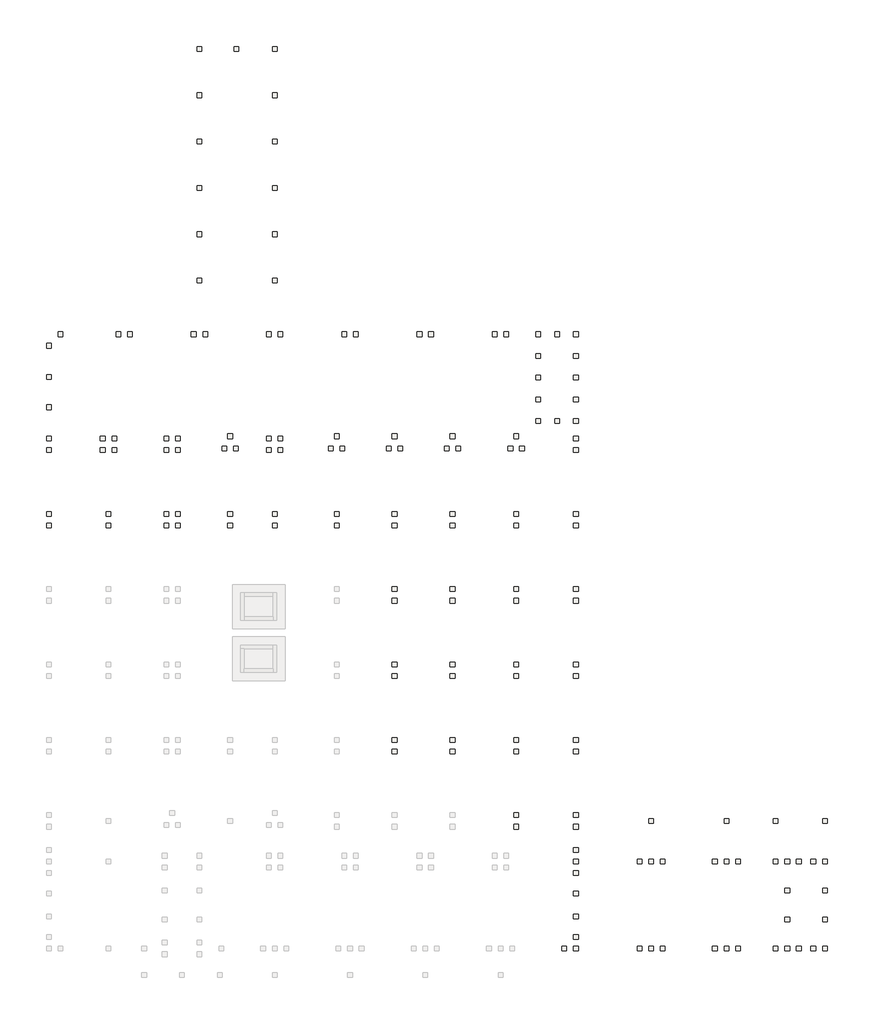
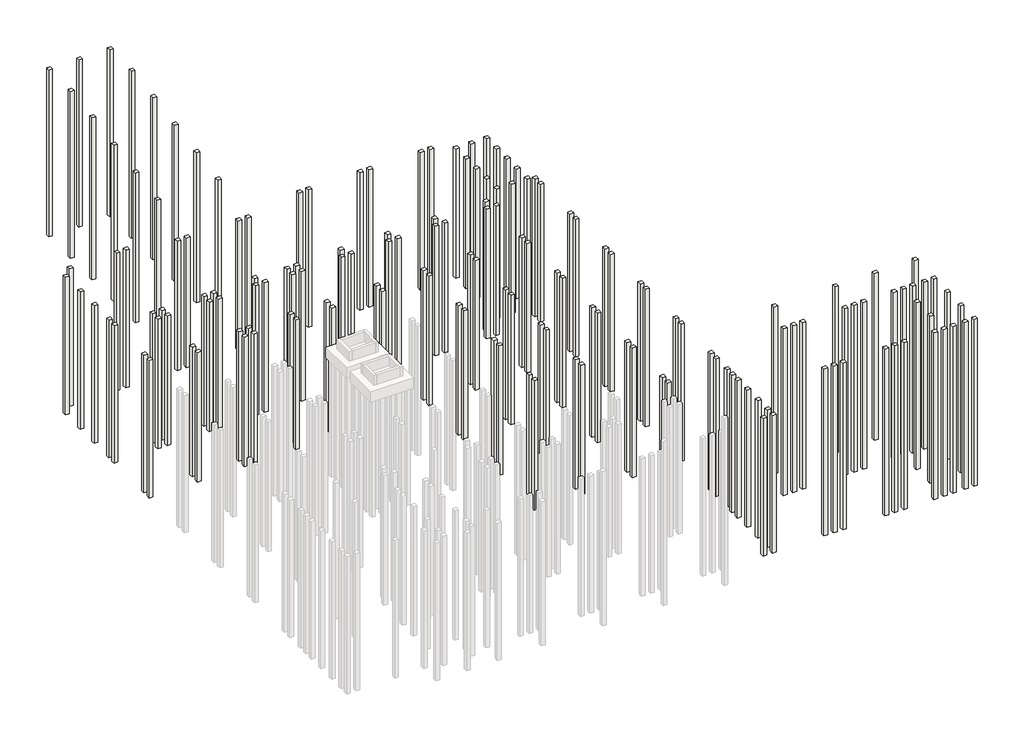
# Not in any storey, part 2 of 2: 160 slabs.
# Revit data of these elements (continued)
# Element 3 (IfcSlab, "NLRS_17_SFO_TLB_funderingspaal geheid beton prefab-AV-MMBPC_gen_rsf : heipaal beton prefab_gen__bxh 400x400") (continued)
#   Materials on its faces: "NLRS_f2_beton prefab_gen_rsf"
# Element 4 (IfcSlab, "NLRS_17_SFO_TLB_funderingspaal geheid beton prefab-AV-MMBPC_gen_rsf : heipaal beton prefab_gen__bxh 400x400")
#   IfcGUID = "10$Kfo5uPCAOPJEOo5LEs3"
#   Slanted Angle = 0.00°
#   NLRS_S_draagvermogen_trek = 0.00 kN
#   NLRS_S_draagvermogen_druk = 0.00 kN
#   Angle = 0.00°
#   IsExternal = yes
#   LoadBearing = yes
#   Slanted = 0
#   Phase Created = NLRS_nieuw
#   Materials on its faces: "NLRS_f2_beton prefab_gen_rsf"
# Element 5 (IfcSlab, "NLRS_17_SFO_TLB_funderingspaal geheid beton prefab-AV-MMBPC_gen_rsf : heipaal beton prefab_gen__bxh 400x400")
#   IfcGUID = "10$Kfo5uPCAOPJEOo5LEsU"
#   Slanted Angle = 0.00°
#   NLRS_S_draagvermogen_trek = 0.00 kN
#   NLRS_S_draagvermogen_druk = 0.00 kN
#   Angle = 0.00°
#   IsExternal = yes
#   LoadBearing = yes
#   Slanted = 0
#   Phase Created = NLRS_nieuw
#   Materials on its faces: "NLRS_f2_beton prefab_gen_rsf"
# Element 6 (IfcSlab, "NLRS_17_SFO_TLB_funderingspaal geheid beton prefab-AV-MMBPC_gen_rsf : heipaal beton prefab_gen__bxh 400x400")
#   IfcGUID = "10$Kfo5uPCAOPJEOo5LEsG"
#   Slanted Angle = 0.00°
#   NLRS_S_draagvermogen_trek = 0.00 kN
#   NLRS_S_draagvermogen_druk = 0.00 kN
#   Angle = 0.00°
#   IsExternal = yes
#   LoadBearing = yes
#   Slanted = 0
#   Phase Created = NLRS_nieuw
#   Materials on its faces: "NLRS_f2_beton prefab_gen_rsf"
# Element 7 (IfcSlab, "NLRS_17_SFO_TLB_funderingspaal geheid beton prefab-AV-MMBPC_gen_rsf : heipaal beton prefab_gen__bxh 400x400")
#   IfcGUID = "10$Kfo5uPCAOPJEOo5LEre"
#   Slanted Angle = 0.00°
#   NLRS_S_draagvermogen_trek = 0.00 kN
#   NLRS_S_draagvermogen_druk = 0.00 kN
#   Angle = 0.00°
#   IsExternal = yes
#   LoadBearing = yes
#   Slanted = 0
#   Phase Created = NLRS_nieuw
#   Materials on its faces: "NLRS_f2_beton prefab_gen_rsf"
# Element 8 (IfcSlab, "NLRS_17_SFO_TLB_funderingspaal geheid beton prefab-AV-MMBPC_gen_rsf : heipaal beton prefab_gen__bxh 400x400")
#   IfcGUID = "10$Kfo5uPCAOPJEOo5LErg"
#   Slanted Angle = 0.00°
#   NLRS_S_draagvermogen_trek = 0.00 kN
#   NLRS_S_draagvermogen_druk = 0.00 kN
#   Angle = 0.00°
#   IsExternal = yes
#   LoadBearing = yes
#   Slanted = 0
#   Phase Created = NLRS_nieuw
#   Materials on its faces: "NLRS_f2_beton prefab_gen_rsf"
# Element 9 (IfcSlab, "NLRS_17_SFO_TLB_funderingspaal geheid beton prefab-AV-MMBPC_gen_rsf : heipaal beton prefab_gen__bxh 400x400")
#   IfcGUID = "10$Kfo5uPCAOPJEOo5LEpb"
#   Slanted Angle = 0.00°
#   NLRS_S_draagvermogen_trek = 0.00 kN
#   NLRS_S_draagvermogen_druk = 0.00 kN
#   Angle = 0.00°
#   IsExternal = yes
#   LoadBearing = yes
#   Slanted = 0
#   Phase Created = NLRS_nieuw
#   Materials on its faces: "NLRS_f2_beton prefab_gen_rsf"
# Element 10 (IfcSlab, "NLRS_17_SFO_TLB_funderingspaal geheid beton prefab-AV-MMBPC_gen_rsf : heipaal beton prefab_gen__bxh 400x400")
#   IfcGUID = "10$Kfo5uPCAOPJEOo5LEpd"
#   Slanted Angle = 0.00°
#   NLRS_S_draagvermogen_trek = 0.00 kN
#   NLRS_S_draagvermogen_druk = 0.00 kN
#   Angle = 0.00°
#   IsExternal = yes
#   LoadBearing = yes
#   Slanted = 0
#   Phase Created = NLRS_nieuw
#   Materials on its faces: "NLRS_f2_beton prefab_gen_rsf"
# Element 11 (IfcSlab, "NLRS_17_SFO_TLB_funderingspaal geheid beton prefab-AV-MMBPC_gen_rsf : heipaal beton prefab_gen__bxh 400x400")
#   IfcGUID = "10$Kfo5uPCAOPJEOo5LEpz"
#   Slanted Angle = 0.00°
#   NLRS_S_draagvermogen_trek = 0.00 kN
#   NLRS_S_draagvermogen_druk = 0.00 kN
#   Angle = 0.00°
#   IsExternal = yes
#   LoadBearing = yes
#   Slanted = 0
#   Phase Created = NLRS_nieuw
#   Materials on its faces: "NLRS_f2_beton prefab_gen_rsf"
# Element 12 (IfcSlab, "NLRS_17_SFO_TLB_funderingspaal geheid beton prefab-AV-MMBPC_gen_rsf : heipaal beton prefab_gen__bxh 400x400")
#   IfcGUID = "10$Kfo5uPCAOPJEOo5LEp$"
#   Slanted Angle = 0.00°
#   NLRS_S_draagvermogen_trek = 0.00 kN
#   NLRS_S_draagvermogen_druk = 0.00 kN
#   Angle = 0.00°
#   IsExternal = yes
#   LoadBearing = yes
#   Slanted = 0
#   Phase Created = NLRS_nieuw
#   Materials on its faces: "NLRS_f2_beton prefab_gen_rsf"
# Element 13 (IfcSlab, "NLRS_17_SFO_TLB_funderingspaal geheid beton prefab-AV-MMBPC_gen_rsf : heipaal beton prefab_gen__bxh 400x400")
#   IfcGUID = "10$Kfo5uPCAOPJEOo5LFTh"
#   Slanted Angle = 0.00°
#   NLRS_S_draagvermogen_trek = 0.00 kN
#   NLRS_S_draagvermogen_druk = 0.00 kN
#   Angle = 0.00°
#   IsExternal = yes
#   LoadBearing = yes
#   Slanted = 0
#   Phase Created = NLRS_nieuw
#   Materials on its faces: "NLRS_f2_beton prefab_gen_rsf"
# Element 14 (IfcSlab, "NLRS_17_SFO_TLB_funderingspaal geheid beton prefab-AV-MMBPC_gen_rsf : heipaal beton prefab_gen__bxh 400x400")
#   IfcGUID = "10$Kfo5uPCAOPJEOo5LFSD"
#   Slanted Angle = 0.00°
#   NLRS_S_draagvermogen_trek = 0.00 kN
#   NLRS_S_draagvermogen_druk = 0.00 kN
#   Angle = 0.00°
#   IsExternal = yes
#   LoadBearing = yes
#   Slanted = 0
#   Phase Created = NLRS_nieuw
#   Materials on its faces: "NLRS_f2_beton prefab_gen_rsf"
# Element 15 (IfcSlab, "NLRS_17_SFO_TLB_funderingspaal geheid beton prefab-AV-MMBPC_gen_rsf : heipaal beton prefab_gen__bxh 400x400")
#   IfcGUID = "10$Kfo5uPCAOPJEOo5LFSk"
#   Slanted Angle = 0.00°
#   NLRS_S_draagvermogen_trek = 0.00 kN
#   NLRS_S_draagvermogen_druk = 0.00 kN
#   Angle = 0.00°
#   IsExternal = yes
#   LoadBearing = yes
#   Slanted = 0
#   Phase Created = NLRS_nieuw
#   Materials on its faces: "NLRS_f2_beton prefab_gen_rsf"
# Element 16 (IfcSlab, "NLRS_17_SFO_TLB_funderingspaal geheid beton prefab-AV-MMBPC_gen_rsf : heipaal beton prefab_gen__bxh 400x400")
#   IfcGUID = "10$Kfo5uPCAOPJEOo5LFSv"
#   Slanted Angle = 0.00°
#   NLRS_S_draagvermogen_trek = 0.00 kN
#   NLRS_S_draagvermogen_druk = 0.00 kN
#   Angle = 0.00°
#   IsExternal = yes
#   LoadBearing = yes
#   Slanted = 0
#   Phase Created = NLRS_nieuw
#   Materials on its faces: "NLRS_f2_beton prefab_gen_rsf"
# Element 17 (IfcSlab, "NLRS_17_SFO_TLB_funderingspaal geheid beton prefab-AV-MMBPC_gen_rsf : heipaal beton prefab_gen__bxh 400x400")
#   IfcGUID = "10$Kfo5uPCAOPJEOo5LFSs"
#   Slanted Angle = 0.00°
#   NLRS_S_draagvermogen_trek = 0.00 kN
#   NLRS_S_draagvermogen_druk = 0.00 kN
#   Angle = 0.00°
#   IsExternal = yes
#   LoadBearing = yes
#   Slanted = 0
#   Phase Created = NLRS_nieuw
#   Materials on its faces: "NLRS_f2_beton prefab_gen_rsf"
# Element 18 (IfcSlab, "NLRS_17_SFO_TLB_funderingspaal geheid beton prefab-AV-MMBPC_gen_rsf : heipaal beton prefab_gen__bxh 400x400")
#   IfcGUID = "10$Kfo5uPCAOPJEOo5LFR1"
#   Slanted Angle = 0.00°
#   NLRS_S_draagvermogen_trek = 0.00 kN
#   NLRS_S_draagvermogen_druk = 0.00 kN
#   Angle = 0.00°
#   IsExternal = yes
#   LoadBearing = yes
#   Slanted = 0
#   Phase Created = NLRS_nieuw
#   Materials on its faces: "NLRS_f2_beton prefab_gen_rsf"
# Element 19 (IfcSlab, "NLRS_17_SFO_TLB_funderingspaal geheid beton prefab-AV-MMBPC_gen_rsf : heipaal beton prefab_gen__bxh 400x400")
#   IfcGUID = "10$Kfo5uPCAOPJEOo5LFQO"
#   Slanted Angle = 0.00°
#   NLRS_S_draagvermogen_trek = 0.00 kN
#   NLRS_S_draagvermogen_druk = 0.00 kN
#   Angle = 0.00°
#   IsExternal = yes
#   LoadBearing = yes
#   Slanted = 0
#   Phase Created = NLRS_nieuw
#   Materials on its faces: "NLRS_f2_beton prefab_gen_rsf"
# Element 20 (IfcSlab, "NLRS_17_SFO_TLB_funderingspaal geheid beton prefab-AV-MMBPC_gen_rsf : heipaal beton prefab_gen__bxh 400x400")
#   IfcGUID = "10$Kfo5uPCAOPJEOo5LFQJ"
#   Slanted Angle = 0.00°
#   NLRS_S_draagvermogen_trek = 0.00 kN
#   NLRS_S_draagvermogen_druk = 0.00 kN
#   Angle = 0.00°
#   IsExternal = yes
#   LoadBearing = yes
#   Slanted = 0
#   Phase Created = NLRS_nieuw
#   Materials on its faces: "NLRS_f2_beton prefab_gen_rsf"
# Element 21 (IfcSlab, "NLRS_17_SFO_TLB_funderingspaal geheid beton prefab-AV-MMBPC_gen_rsf : heipaal beton prefab_gen__bxh 400x400")
#   IfcGUID = "10$Kfo5uPCAOPJEOo5LFQk"
#   Slanted Angle = 0.00°
#   NLRS_S_draagvermogen_trek = 0.00 kN
#   NLRS_S_draagvermogen_druk = 0.00 kN
#   Angle = 0.00°
#   IsExternal = yes
#   LoadBearing = yes
#   Slanted = 0
#   Phase Created = NLRS_nieuw
#   Materials on its faces: "NLRS_f2_beton prefab_gen_rsf"
# Element 22 (IfcSlab, "NLRS_17_SFO_TLB_funderingspaal geheid beton prefab-AV-MMBPC_gen_rsf : heipaal beton prefab_gen__bxh 400x400")
#   IfcGUID = "10$Kfo5uPCAOPJEOo5LFPx"
#   Slanted Angle = 0.00°
#   NLRS_S_draagvermogen_trek = 0.00 kN
#   NLRS_S_draagvermogen_druk = 0.00 kN
#   Angle = 0.00°
#   IsExternal = yes
#   LoadBearing = yes
#   Slanted = 0
#   Phase Created = NLRS_nieuw
#   Materials on its faces: "NLRS_f2_beton prefab_gen_rsf"
# Element 23 (IfcSlab, "NLRS_17_SFO_TLB_funderingspaal geheid beton prefab-AV-MMBPC_gen_rsf : heipaal beton prefab_gen__bxh 400x400")
#   IfcGUID = "10$Kfo5uPCAOPJEOo5LFOK"
#   Slanted Angle = 0.00°
#   NLRS_S_draagvermogen_trek = 0.00 kN
#   NLRS_S_draagvermogen_druk = 0.00 kN
#   Angle = 0.00°
#   IsExternal = yes
#   LoadBearing = yes
#   Slanted = 0
#   Phase Created = NLRS_nieuw
#   Materials on its faces: "NLRS_f2_beton prefab_gen_rsf"
# Element 24 (IfcSlab, "NLRS_17_SFO_TLB_funderingspaal geheid beton prefab-AV-MMBPC_gen_rsf : heipaal beton prefab_gen__bxh 400x400")
#   IfcGUID = "10$Kfo5uPCAOPJEOo5LFOl"
#   Slanted Angle = 0.00°
#   NLRS_S_draagvermogen_trek = 0.00 kN
#   NLRS_S_draagvermogen_druk = 0.00 kN
#   Angle = 0.00°
#   IsExternal = yes
#   LoadBearing = yes
#   Slanted = 0
#   Phase Created = NLRS_nieuw
#   Materials on its faces: "NLRS_f2_beton prefab_gen_rsf"
# Element 25 (IfcSlab, "NLRS_17_SFO_TLB_funderingspaal geheid beton prefab-AV-MMBPC_gen_rsf : heipaal beton prefab_gen__bxh 400x400")
#   IfcGUID = "3loy75XKz2Rw4dS8JWiamE"
#   Slanted Angle = 0.00°
#   NLRS_S_draagvermogen_trek = 0.00 kN
#   NLRS_S_draagvermogen_druk = 0.00 kN
#   Angle = 0.00°
#   IsExternal = yes
#   LoadBearing = yes
#   Slanted = 0
#   Phase Created = NLRS_nieuw
#   Materials on its faces: "NLRS_f2_beton prefab_gen_rsf"
# Element 26 (IfcSlab, "NLRS_17_SFO_TLB_funderingspaal geheid beton prefab-AV-MMBPC_gen_rsf : heipaal beton prefab_gen__bxh 400x400")
#   IfcGUID = "3loy75XKz2Rw4dS8JWiamC"
#   Slanted Angle = 0.00°
#   NLRS_S_draagvermogen_trek = 0.00 kN
#   NLRS_S_draagvermogen_druk = 0.00 kN
#   Angle = 0.00°
#   IsExternal = yes
#   LoadBearing = yes
#   Slanted = 0
#   Phase Created = NLRS_nieuw
#   Materials on its faces: "NLRS_f2_beton prefab_gen_rsf"
# Element 27 (IfcSlab, "NLRS_17_SFO_TLB_funderingspaal geheid beton prefab-AV-MMBPC_gen_rsf : heipaal beton prefab_gen__bxh 400x400")
#   IfcGUID = "3loy75XKz2Rw4dS8JWiamv"
#   Slanted Angle = 0.00°
#   NLRS_S_draagvermogen_trek = 0.00 kN
#   NLRS_S_draagvermogen_druk = 0.00 kN
#   Angle = 0.00°
#   IsExternal = yes
#   LoadBearing = yes
#   Slanted = 0
#   Phase Created = NLRS_nieuw
#   Materials on its faces: "NLRS_f2_beton prefab_gen_rsf"
# Element 28 (IfcSlab, "NLRS_17_SFO_TLB_funderingspaal geheid beton prefab-AV-MMBPC_gen_rsf : heipaal beton prefab_gen__bxh 400x400")
#   IfcGUID = "3loy75XKz2Rw4dS8JWiam$"
#   Slanted Angle = 0.00°
#   NLRS_S_draagvermogen_trek = 0.00 kN
#   NLRS_S_draagvermogen_druk = 0.00 kN
#   Angle = 0.00°
#   IsExternal = yes
#   LoadBearing = yes
#   Slanted = 0
#   Phase Created = NLRS_nieuw
#   Materials on its faces: "NLRS_f2_beton prefab_gen_rsf"
# Element 29 (IfcSlab, "NLRS_17_SFO_TLB_funderingspaal geheid beton prefab-AV-MMBPC_gen_rsf : heipaal beton prefab_gen__bxh 400x400")
#   IfcGUID = "3loy75XKz2Rw4dS8JWiama"
#   Slanted Angle = 0.00°
#   NLRS_S_draagvermogen_trek = 0.00 kN
#   NLRS_S_draagvermogen_druk = 0.00 kN
#   Angle = 0.00°
#   IsExternal = yes
#   LoadBearing = yes
#   Slanted = 0
#   Phase Created = NLRS_nieuw
#   Materials on its faces: "NLRS_f2_beton prefab_gen_rsf"
# Element 30 (IfcSlab, "NLRS_17_SFO_TLB_funderingspaal geheid beton prefab-AV-MMBPC_gen_rsf : heipaal beton prefab_gen__bxh 400x400")
#   IfcGUID = "3loy75XKz2Rw4dS8JWiamg"
#   Slanted Angle = 0.00°
#   NLRS_S_draagvermogen_trek = 0.00 kN
#   NLRS_S_draagvermogen_druk = 0.00 kN
#   Angle = 0.00°
#   IsExternal = yes
#   LoadBearing = yes
#   Slanted = 0
#   Phase Created = NLRS_nieuw
#   Materials on its faces: "NLRS_f2_beton prefab_gen_rsf"
# Element 31 (IfcSlab, "NLRS_17_SFO_TLB_funderingspaal geheid beton prefab-AV-MMBPC_gen_rsf : heipaal beton prefab_gen__bxh 400x400")
#   IfcGUID = "3loy75XKz2Rw4dS8JWiapN"
#   Slanted Angle = 0.00°
#   NLRS_S_draagvermogen_trek = 0.00 kN
#   NLRS_S_draagvermogen_druk = 0.00 kN
#   Angle = 0.00°
#   IsExternal = yes
#   LoadBearing = yes
#   Slanted = 0
#   Phase Created = NLRS_nieuw
#   Materials on its faces: "NLRS_f2_beton prefab_gen_rsf"
# Element 32 (IfcSlab, "NLRS_17_SFO_TLB_funderingspaal geheid beton prefab-AV-MMBPC_gen_rsf : heipaal beton prefab_gen__bxh 400x400")
#   IfcGUID = "3loy75XKz2Rw4dS8JWiapL"
#   Slanted Angle = 0.00°
#   NLRS_S_draagvermogen_trek = 0.00 kN
#   NLRS_S_draagvermogen_druk = 0.00 kN
#   Angle = 0.00°
#   IsExternal = yes
#   LoadBearing = yes
#   Slanted = 0
#   Phase Created = NLRS_nieuw
#   Materials on its faces: "NLRS_f2_beton prefab_gen_rsf"
# Element 33 (IfcSlab, "NLRS_17_SFO_TLB_funderingspaal geheid beton prefab-AV-MMBPC_gen_rsf : heipaal beton prefab_gen__bxh 400x400")
#   IfcGUID = "3loy75XKz2Rw4dS8JWiap2"
#   Slanted Angle = 0.00°
#   NLRS_S_draagvermogen_trek = 0.00 kN
#   NLRS_S_draagvermogen_druk = 0.00 kN
#   Angle = 0.00°
#   IsExternal = yes
#   LoadBearing = yes
#   Slanted = 0
#   Phase Created = NLRS_nieuw
#   Materials on its faces: "NLRS_f2_beton prefab_gen_rsf"
# Element 34 (IfcSlab, "NLRS_17_SFO_TLB_funderingspaal geheid beton prefab-AV-MMBPC_gen_rsf : heipaal beton prefab_gen__bxh 400x400")
#   IfcGUID = "3loy75XKz2Rw4dS8JWiap0"
#   Slanted Angle = 0.00°
#   NLRS_S_draagvermogen_trek = 0.00 kN
#   NLRS_S_draagvermogen_druk = 0.00 kN
#   Angle = 0.00°
#   IsExternal = yes
#   LoadBearing = yes
#   Slanted = 0
#   Phase Created = NLRS_nieuw
#   Materials on its faces: "NLRS_f2_beton prefab_gen_rsf"
# Element 35 (IfcSlab, "NLRS_17_SFO_TLB_funderingspaal geheid beton prefab-AV-MMBPC_gen_rsf : heipaal beton prefab_gen__bxh 400x400")
#   IfcGUID = "3loy75XKz2Rw4dS8JWiapD"
#   Slanted Angle = 0.00°
#   NLRS_S_draagvermogen_trek = 0.00 kN
#   NLRS_S_draagvermogen_druk = 0.00 kN
#   Angle = 0.00°
#   IsExternal = yes
#   LoadBearing = yes
#   Slanted = 0
#   Phase Created = NLRS_nieuw
#   Materials on its faces: "NLRS_f2_beton prefab_gen_rsf"
# Element 36 (IfcSlab, "NLRS_17_SFO_TLB_funderingspaal geheid beton prefab-AV-MMBPC_gen_rsf : heipaal beton prefab_gen__bxh 400x400")
#   IfcGUID = "3loy75XKz2Rw4dS8JWiapp"
#   Slanted Angle = 0.00°
#   NLRS_S_draagvermogen_trek = 0.00 kN
#   NLRS_S_draagvermogen_druk = 0.00 kN
#   Angle = 0.00°
#   IsExternal = yes
#   LoadBearing = yes
#   Slanted = 0
#   Phase Created = NLRS_nieuw
#   Materials on its faces: "NLRS_f2_beton prefab_gen_rsf"
# Element 37 (IfcSlab, "NLRS_17_SFO_TLB_funderingspaal geheid beton prefab-AV-MMBPC_gen_rsf : heipaal beton prefab_gen__bxh 400x400")
#   IfcGUID = "3loy75XKz2Rw4dS8JWiao6"
#   Slanted Angle = 0.00°
#   NLRS_S_draagvermogen_trek = 0.00 kN
#   NLRS_S_draagvermogen_druk = 0.00 kN
#   Angle = 0.00°
#   IsExternal = yes
#   LoadBearing = yes
#   Slanted = 0
#   Phase Created = NLRS_nieuw
#   Materials on its faces: "NLRS_f2_beton prefab_gen_rsf"
# Element 38 (IfcSlab, "NLRS_17_SFO_TLB_funderingspaal geheid beton prefab-AV-MMBPC_gen_rsf : heipaal beton prefab_gen__bxh 400x400")
#   IfcGUID = "3loy75XKz2Rw4dS8JWiao4"
#   Slanted Angle = 0.00°
#   NLRS_S_draagvermogen_trek = 0.00 kN
#   NLRS_S_draagvermogen_druk = 0.00 kN
#   Angle = 0.00°
#   IsExternal = yes
#   LoadBearing = yes
#   Slanted = 0
#   Phase Created = NLRS_nieuw
#   Materials on its faces: "NLRS_f2_beton prefab_gen_rsf"
# Element 39 (IfcSlab, "NLRS_17_SFO_TLB_funderingspaal geheid beton prefab-AV-MMBPC_gen_rsf : heipaal beton prefab_gen__bxh 400x400")
#   IfcGUID = "3loy75XKz2Rw4dS8JWiaon"
#   Slanted Angle = 0.00°
#   NLRS_S_draagvermogen_trek = 0.00 kN
#   NLRS_S_draagvermogen_druk = 0.00 kN
#   Angle = 0.00°
#   IsExternal = yes
#   LoadBearing = yes
#   Slanted = 0
#   Phase Created = NLRS_nieuw
#   Materials on its faces: "NLRS_f2_beton prefab_gen_rsf"
# Element 40 (IfcSlab, "NLRS_17_SFO_TLB_funderingspaal geheid beton prefab-AV-MMBPC_gen_rsf : heipaal beton prefab_gen__bxh 400x400")
#   IfcGUID = "3loy75XKz2Rw4dS8JWiaot"
#   Slanted Angle = 0.00°
#   NLRS_S_draagvermogen_trek = 0.00 kN
#   NLRS_S_draagvermogen_druk = 0.00 kN
#   Angle = 0.00°
#   IsExternal = yes
#   LoadBearing = yes
#   Slanted = 0
#   Phase Created = NLRS_nieuw
#   Materials on its faces: "NLRS_f2_beton prefab_gen_rsf"
# Element 41 (IfcSlab, "NLRS_17_SFO_TLB_funderingspaal geheid beton prefab-AV-MMBPC_gen_rsf : heipaal beton prefab_gen__bxh 400x400")
#   IfcGUID = "3loy75XKz2Rw4dS8JWiaoy"
#   Slanted Angle = 0.00°
#   NLRS_S_draagvermogen_trek = 0.00 kN
#   NLRS_S_draagvermogen_druk = 0.00 kN
#   Angle = 0.00°
#   IsExternal = yes
#   LoadBearing = yes
#   Slanted = 0
#   Phase Created = NLRS_nieuw
#   Materials on its faces: "NLRS_f2_beton prefab_gen_rsf"
# Element 42 (IfcSlab, "NLRS_17_SFO_TLB_funderingspaal geheid beton prefab-AV-MMBPC_gen_rsf : heipaal beton prefab_gen__bxh 400x400")
#   IfcGUID = "3loy75XKz2Rw4dS8JWiaoY"
#   Slanted Angle = 0.00°
#   NLRS_S_draagvermogen_trek = 0.00 kN
#   NLRS_S_draagvermogen_druk = 0.00 kN
#   Angle = 0.00°
#   IsExternal = yes
#   LoadBearing = yes
#   Slanted = 0
#   Phase Created = NLRS_nieuw
#   Materials on its faces: "NLRS_f2_beton prefab_gen_rsf"
# Element 43 (IfcSlab, "NLRS_17_SFO_TLB_funderingspaal geheid beton prefab-AV-MMBPC_gen_rsf : heipaal beton prefab_gen__bxh 400x400")
#   IfcGUID = "3loy75XKz2Rw4dS8JWiaol"
#   Slanted Angle = 0.00°
#   NLRS_S_draagvermogen_trek = 0.00 kN
#   NLRS_S_draagvermogen_druk = 0.00 kN
#   Angle = 0.00°
#   IsExternal = yes
#   LoadBearing = yes
#   Slanted = 0
#   Phase Created = NLRS_nieuw
#   Materials on its faces: "NLRS_f2_beton prefab_gen_rsf"
# Element 44 (IfcSlab, "NLRS_17_SFO_TLB_funderingspaal geheid beton prefab-AV-MMBPC_gen_rsf : heipaal beton prefab_gen__bxh 400x400")
#   IfcGUID = "3loy75XKz2Rw4dS8JWiaoj"
#   Slanted Angle = 0.00°
#   NLRS_S_draagvermogen_trek = 0.00 kN
#   NLRS_S_draagvermogen_druk = 0.00 kN
#   Angle = 0.00°
#   IsExternal = yes
#   LoadBearing = yes
#   Slanted = 0
#   Phase Created = NLRS_nieuw
#   Materials on its faces: "NLRS_f2_beton prefab_gen_rsf"
# Element 45 (IfcSlab, "NLRS_17_SFO_TLB_funderingspaal geheid beton prefab-AV-MMBPC_gen_rsf : heipaal beton prefab_gen__bxh 400x400")
#   IfcGUID = "3loy75XKz2Rw4dS8JWiarQ"
#   Slanted Angle = 0.00°
#   NLRS_S_draagvermogen_trek = 0.00 kN
#   NLRS_S_draagvermogen_druk = 0.00 kN
#   Angle = 0.00°
#   IsExternal = yes
#   LoadBearing = yes
#   Slanted = 0
#   Phase Created = NLRS_nieuw
#   Materials on its faces: "NLRS_f2_beton prefab_gen_rsf"
# Element 46 (IfcSlab, "NLRS_17_SFO_TLB_funderingspaal geheid beton prefab-AV-MMBPC_gen_rsf : heipaal beton prefab_gen__bxh 400x400")
#   IfcGUID = "3loy75XKz2Rw4dS8JWiarO"
#   Slanted Angle = 0.00°
#   NLRS_S_draagvermogen_trek = 0.00 kN
#   NLRS_S_draagvermogen_druk = 0.00 kN
#   Angle = 0.00°
#   IsExternal = yes
#   LoadBearing = yes
#   Slanted = 0
#   Phase Created = NLRS_nieuw
#   Materials on its faces: "NLRS_f2_beton prefab_gen_rsf"
# Element 47 (IfcSlab, "NLRS_17_SFO_TLB_funderingspaal geheid beton prefab-AV-MMBPC_gen_rsf : heipaal beton prefab_gen__bxh 400x400")
#   IfcGUID = "3loy75XKz2Rw4dS8JWiar5"
#   Slanted Angle = 0.00°
#   NLRS_S_draagvermogen_trek = 0.00 kN
#   NLRS_S_draagvermogen_druk = 0.00 kN
#   Angle = 0.00°
#   IsExternal = yes
#   LoadBearing = yes
#   Slanted = 0
#   Phase Created = NLRS_nieuw
#   Materials on its faces: "NLRS_f2_beton prefab_gen_rsf"
# Element 48 (IfcSlab, "NLRS_17_SFO_TLB_funderingspaal geheid beton prefab-AV-MMBPC_gen_rsf : heipaal beton prefab_gen__bxh 400x400")
#   IfcGUID = "3loy75XKz2Rw4dS8JWiarB"
#   Slanted Angle = 0.00°
#   NLRS_S_draagvermogen_trek = 0.00 kN
#   NLRS_S_draagvermogen_druk = 0.00 kN
#   Angle = 0.00°
#   IsExternal = yes
#   LoadBearing = yes
#   Slanted = 0
#   Phase Created = NLRS_nieuw
#   Materials on its faces: "NLRS_f2_beton prefab_gen_rsf"
# Element 49 (IfcSlab, "NLRS_17_SFO_TLB_funderingspaal geheid beton prefab-AV-MMBPC_gen_rsf : heipaal beton prefab_gen__bxh 400x400")
#   IfcGUID = "3loy75XKz2Rw4dS8JWiarm"
#   Slanted Angle = 0.00°
#   NLRS_S_draagvermogen_trek = 0.00 kN
#   NLRS_S_draagvermogen_druk = 0.00 kN
#   Angle = 0.00°
#   IsExternal = yes
#   LoadBearing = yes
#   Slanted = 0
#   Phase Created = NLRS_nieuw
#   Materials on its faces: "NLRS_f2_beton prefab_gen_rsf"
# Element 50 (IfcSlab, "NLRS_17_SFO_TLB_funderingspaal geheid beton prefab-AV-MMBPC_gen_rsf : heipaal beton prefab_gen__bxh 400x400")
#   IfcGUID = "3loy75XKz2Rw4dS8JWiars"
#   Slanted Angle = 0.00°
#   NLRS_S_draagvermogen_trek = 0.00 kN
#   NLRS_S_draagvermogen_druk = 0.00 kN
#   Angle = 0.00°
#   IsExternal = yes
#   LoadBearing = yes
#   Slanted = 0
#   Phase Created = NLRS_nieuw
#   Materials on its faces: "NLRS_f2_beton prefab_gen_rsf"
# Element 51 (IfcSlab, "NLRS_17_SFO_TLB_funderingspaal geheid beton prefab-AV-MMBPC_gen_rsf : heipaal beton prefab_gen__bxh 400x400")
#   IfcGUID = "3loy75XKz2Rw4dS8JWia96"
#   Slanted Angle = 0.00°
#   NLRS_S_draagvermogen_trek = 0.00 kN
#   NLRS_S_draagvermogen_druk = 0.00 kN
#   Angle = 0.00°
#   IsExternal = yes
#   LoadBearing = yes
#   Slanted = 0
#   Phase Created = NLRS_nieuw
#   Materials on its faces: "NLRS_f2_beton prefab_gen_rsf"
# Element 52 (IfcSlab, "NLRS_17_SFO_TLB_funderingspaal geheid beton prefab-AV-MMBPC_gen_rsf : heipaal beton prefab_gen__bxh 400x400")
#   IfcGUID = "3loy75XKz2Rw4dS8JWia94"
#   Slanted Angle = 0.00°
#   NLRS_S_draagvermogen_trek = 0.00 kN
#   NLRS_S_draagvermogen_druk = 0.00 kN
#   Angle = 0.00°
#   IsExternal = yes
#   LoadBearing = yes
#   Slanted = 0
#   Phase Created = NLRS_nieuw
#   Materials on its faces: "NLRS_f2_beton prefab_gen_rsf"
# Element 53 (IfcSlab, "NLRS_17_SFO_TLB_funderingspaal geheid beton prefab-AV-MMBPC_gen_rsf : heipaal beton prefab_gen__bxh 400x400")
#   IfcGUID = "3loy75XKz2Rw4dS8JWia9A"
#   Slanted Angle = 0.00°
#   NLRS_S_draagvermogen_trek = 0.00 kN
#   NLRS_S_draagvermogen_druk = 0.00 kN
#   Angle = 0.00°
#   IsExternal = yes
#   LoadBearing = yes
#   Slanted = 0
#   Phase Created = NLRS_nieuw
#   Materials on its faces: "NLRS_f2_beton prefab_gen_rsf"
# Element 54 (IfcSlab, "NLRS_17_SFO_TLB_funderingspaal geheid beton prefab-AV-MMBPC_gen_rsf : heipaal beton prefab_gen__bxh 400x400")
#   IfcGUID = "3loy75XKz2Rw4dS8JWia98"
#   Slanted Angle = 0.00°
#   NLRS_S_draagvermogen_trek = 0.00 kN
#   NLRS_S_draagvermogen_druk = 0.00 kN
#   Angle = 0.00°
#   IsExternal = yes
#   LoadBearing = yes
#   Slanted = 0
#   Phase Created = NLRS_nieuw
#   Materials on its faces: "NLRS_f2_beton prefab_gen_rsf"
# Element 55 (IfcSlab, "NLRS_17_SFO_TLB_funderingspaal geheid beton prefab-AV-MMBPC_gen_rsf : heipaal beton prefab_gen__bxh 400x400")
#   IfcGUID = "3loy75XKz2Rw4dS8JWia9l"
#   Slanted Angle = 0.00°
#   NLRS_S_draagvermogen_trek = 0.00 kN
#   NLRS_S_draagvermogen_druk = 0.00 kN
#   Angle = 0.00°
#   IsExternal = yes
#   LoadBearing = yes
#   Slanted = 0
#   Phase Created = NLRS_nieuw
#   Materials on its faces: "NLRS_f2_beton prefab_gen_rsf"
# Element 56 (IfcSlab, "NLRS_17_SFO_TLB_funderingspaal geheid beton prefab-AV-MMBPC_gen_rsf : heipaal beton prefab_gen__bxh 400x400")
#   IfcGUID = "3loy75XKz2Rw4dS8JWia9j"
#   Slanted Angle = 0.00°
#   NLRS_S_draagvermogen_trek = 0.00 kN
#   NLRS_S_draagvermogen_druk = 0.00 kN
#   Angle = 0.00°
#   IsExternal = yes
#   LoadBearing = yes
#   Slanted = 0
#   Phase Created = NLRS_nieuw
#   Materials on its faces: "NLRS_f2_beton prefab_gen_rsf"
# Element 57 (IfcSlab, "NLRS_17_SFO_TLB_funderingspaal geheid beton prefab-AV-MMBPC_gen_rsf : heipaal beton prefab_gen__bxh 400x400")
#   IfcGUID = "3loy75XKz2Rw4dS8JWia8J"
#   Slanted Angle = 0.00°
#   NLRS_S_draagvermogen_trek = 0.00 kN
#   NLRS_S_draagvermogen_druk = 0.00 kN
#   Angle = 0.00°
#   IsExternal = yes
#   LoadBearing = yes
#   Slanted = 0
#   Phase Created = NLRS_nieuw
#   Materials on its faces: "NLRS_f2_beton prefab_gen_rsf"
# Element 58 (IfcSlab, "NLRS_17_SFO_TLB_funderingspaal geheid beton prefab-AV-MMBPC_gen_rsf : heipaal beton prefab_gen__bxh 400x400")
#   IfcGUID = "3loy75XKz2Rw4dS8JWia8H"
#   Slanted Angle = 0.00°
#   NLRS_S_draagvermogen_trek = 0.00 kN
#   NLRS_S_draagvermogen_druk = 0.00 kN
#   Angle = 0.00°
#   IsExternal = yes
#   LoadBearing = yes
#   Slanted = 0
#   Phase Created = NLRS_nieuw
#   Materials on its faces: "NLRS_f2_beton prefab_gen_rsf"
# Element 59 (IfcSlab, "NLRS_17_SFO_TLB_funderingspaal geheid beton prefab-AV-MMBPC_gen_rsf : heipaal beton prefab_gen__bxh 400x400")
#   IfcGUID = "3loy75XKz2Rw4dS8JWia8q"
#   Slanted Angle = 0.00°
#   NLRS_S_draagvermogen_trek = 0.00 kN
#   NLRS_S_draagvermogen_druk = 0.00 kN
#   Angle = 0.00°
#   IsExternal = yes
#   LoadBearing = yes
#   Slanted = 0
#   Phase Created = NLRS_nieuw
#   Materials on its faces: "NLRS_f2_beton prefab_gen_rsf"
# Element 60 (IfcSlab, "NLRS_17_SFO_TLB_funderingspaal geheid beton prefab-AV-MMBPC_gen_rsf : heipaal beton prefab_gen__bxh 400x400")
#   IfcGUID = "3loy75XKz2Rw4dS8JWia8w"
#   Slanted Angle = 0.00°
#   NLRS_S_draagvermogen_trek = 0.00 kN
#   NLRS_S_draagvermogen_druk = 0.00 kN
#   Angle = 0.00°
#   IsExternal = yes
#   LoadBearing = yes
#   Slanted = 0
#   Phase Created = NLRS_nieuw
#   Materials on its faces: "NLRS_f2_beton prefab_gen_rsf"
# Element 61 (IfcSlab, "NLRS_17_SFO_TLB_funderingspaal geheid beton prefab-AV-MMBPC_gen_rsf : heipaal beton prefab_gen__bxh 400x400")
#   IfcGUID = "3loy75XKz2Rw4dS8JWia8u"
#   Slanted Angle = 0.00°
#   NLRS_S_draagvermogen_trek = 0.00 kN
#   NLRS_S_draagvermogen_druk = 0.00 kN
#   Angle = 0.00°
#   IsExternal = yes
#   LoadBearing = yes
#   Slanted = 0
#   Phase Created = NLRS_nieuw
#   Materials on its faces: "NLRS_f2_beton prefab_gen_rsf"
# Element 62 (IfcSlab, "NLRS_17_SFO_TLB_funderingspaal geheid beton prefab-AV-MMBPC_gen_rsf : heipaal beton prefab_gen__bxh 400x400")
#   IfcGUID = "3loy75XKz2Rw4dS8JWiaDh"
#   Slanted Angle = 0.00°
#   NLRS_S_draagvermogen_trek = 0.00 kN
#   NLRS_S_draagvermogen_druk = 0.00 kN
#   Angle = 0.00°
#   IsExternal = yes
#   LoadBearing = yes
#   Slanted = 0
#   Phase Created = NLRS_nieuw
#   Materials on its faces: "NLRS_f2_beton prefab_gen_rsf"
# Element 63 (IfcSlab, "NLRS_17_SFO_TLB_funderingspaal geheid beton prefab-AV-MMBPC_gen_rsf : heipaal beton prefab_gen__bxh 400x400")
#   IfcGUID = "3loy75XKz2Rw4dS8JWiaDf"
#   Slanted Angle = 0.00°
#   NLRS_S_draagvermogen_trek = 0.00 kN
#   NLRS_S_draagvermogen_druk = 0.00 kN
#   Angle = 0.00°
#   IsExternal = yes
#   LoadBearing = yes
#   Slanted = 0
#   Phase Created = NLRS_nieuw
#   Materials on its faces: "NLRS_f2_beton prefab_gen_rsf"
# Element 64 (IfcSlab, "NLRS_17_SFO_TLB_funderingspaal geheid beton prefab-AV-MMBPC_gen_rsf : heipaal beton prefab_gen__bxh 400x400")
#   IfcGUID = "3loy75XKz2Rw4dS8JWiaDl"
#   Slanted Angle = 0.00°
#   NLRS_S_draagvermogen_trek = 0.00 kN
#   NLRS_S_draagvermogen_druk = 0.00 kN
#   Angle = 0.00°
#   IsExternal = yes
#   LoadBearing = yes
#   Slanted = 0
#   Phase Created = NLRS_nieuw
#   Materials on its faces: "NLRS_f2_beton prefab_gen_rsf"
# Element 65 (IfcSlab, "NLRS_17_SFO_TLB_funderingspaal geheid beton prefab-AV-MMBPC_gen_rsf : heipaal beton prefab_gen__bxh 400x400")
#   IfcGUID = "3loy75XKz2Rw4dS8JWiaDj"
#   Slanted Angle = 0.00°
#   NLRS_S_draagvermogen_trek = 0.00 kN
#   NLRS_S_draagvermogen_druk = 0.00 kN
#   Angle = 0.00°
#   IsExternal = yes
#   LoadBearing = yes
#   Slanted = 0
#   Phase Created = NLRS_nieuw
#   Materials on its faces: "NLRS_f2_beton prefab_gen_rsf"
# Element 66 (IfcSlab, "NLRS_17_SFO_TLB_funderingspaal geheid beton prefab-AV-MMBPC_gen_rsf : heipaal beton prefab_gen__bxh 400x400")
#   IfcGUID = "3loy75XKz2Rw4dS8JWiaC7"
#   Slanted Angle = 0.00°
#   NLRS_S_draagvermogen_trek = 0.00 kN
#   NLRS_S_draagvermogen_druk = 0.00 kN
#   Angle = 0.00°
#   IsExternal = yes
#   LoadBearing = yes
#   Slanted = 0
#   Phase Created = NLRS_nieuw
#   Materials on its faces: "NLRS_f2_beton prefab_gen_rsf"
# Element 67 (IfcSlab, "NLRS_17_SFO_TLB_funderingspaal geheid beton prefab-AV-MMBPC_gen_rsf : heipaal beton prefab_gen__bxh 400x400")
#   IfcGUID = "3loy75XKz2Rw4dS8JWiaC5"
#   Slanted Angle = 0.00°
#   NLRS_S_draagvermogen_trek = 0.00 kN
#   NLRS_S_draagvermogen_druk = 0.00 kN
#   Angle = 0.00°
#   IsExternal = yes
#   LoadBearing = yes
#   Slanted = 0
#   Phase Created = NLRS_nieuw
#   Materials on its faces: "NLRS_f2_beton prefab_gen_rsf"
# Element 68 (IfcSlab, "NLRS_17_SFO_TLB_funderingspaal geheid beton prefab-AV-MMBPC_gen_rsf : heipaal beton prefab_gen__bxh 400x400")
#   IfcGUID = "3loy75XKz2Rw4dS8JWiaCB"
#   Slanted Angle = 0.00°
#   NLRS_S_draagvermogen_trek = 0.00 kN
#   NLRS_S_draagvermogen_druk = 0.00 kN
#   Angle = 0.00°
#   IsExternal = yes
#   LoadBearing = yes
#   Slanted = 0
#   Phase Created = NLRS_nieuw
#   Materials on its faces: "NLRS_f2_beton prefab_gen_rsf"
# Element 69 (IfcSlab, "NLRS_17_SFO_TLB_funderingspaal geheid beton prefab-AV-MMBPC_gen_rsf : heipaal beton prefab_gen__bxh 400x400")
#   IfcGUID = "3loy75XKz2Rw4dS8JWiaCs"
#   Slanted Angle = 0.00°
#   NLRS_S_draagvermogen_trek = 0.00 kN
#   NLRS_S_draagvermogen_druk = 0.00 kN
#   Angle = 0.00°
#   IsExternal = yes
#   LoadBearing = yes
#   Slanted = 0
#   Phase Created = NLRS_nieuw
#   Materials on its faces: "NLRS_f2_beton prefab_gen_rsf"
# Element 70 (IfcSlab, "NLRS_17_SFO_TLB_funderingspaal geheid beton prefab-AV-MMBPC_gen_rsf : heipaal beton prefab_gen__bxh 400x400")
#   IfcGUID = "3loy75XKz2Rw4dS8JWiaCq"
#   Slanted Angle = 0.00°
#   NLRS_S_draagvermogen_trek = 0.00 kN
#   NLRS_S_draagvermogen_druk = 0.00 kN
#   Angle = 0.00°
#   IsExternal = yes
#   LoadBearing = yes
#   Slanted = 0
#   Phase Created = NLRS_nieuw
#   Materials on its faces: "NLRS_f2_beton prefab_gen_rsf"
# Element 71 (IfcSlab, "NLRS_17_SFO_TLB_funderingspaal geheid beton prefab-AV-MMBPC_gen_rsf : heipaal beton prefab_gen__bxh 400x400")
#   IfcGUID = "3loy75XKz2Rw4dS8JWiaCw"
#   Slanted Angle = 0.00°
#   NLRS_S_draagvermogen_trek = 0.00 kN
#   NLRS_S_draagvermogen_druk = 0.00 kN
#   Angle = 0.00°
#   IsExternal = yes
#   LoadBearing = yes
#   Slanted = 0
#   Phase Created = NLRS_nieuw
#   Materials on its faces: "NLRS_f2_beton prefab_gen_rsf"
# Element 72 (IfcSlab, "NLRS_17_SFO_TLB_funderingspaal geheid beton prefab-AV-MMBPC_gen_rsf : heipaal beton prefab_gen__bxh 400x400")
#   IfcGUID = "3loy75XKz2Rw4dS8JWiaCb"
#   Slanted Angle = 0.00°
#   NLRS_S_draagvermogen_trek = 0.00 kN
#   NLRS_S_draagvermogen_druk = 0.00 kN
#   Angle = 0.00°
#   IsExternal = yes
#   LoadBearing = yes
#   Slanted = 0
#   Phase Created = NLRS_nieuw
#   Materials on its faces: "NLRS_f2_beton prefab_gen_rsf"
# Element 73 (IfcSlab, "NLRS_17_SFO_TLB_funderingspaal geheid beton prefab-AV-MMBPC_gen_rsf : heipaal beton prefab_gen__bxh 400x400")
#   IfcGUID = "3loy75XKz2Rw4dS8JWiaCh"
#   Slanted Angle = 0.00°
#   NLRS_S_draagvermogen_trek = 0.00 kN
#   NLRS_S_draagvermogen_druk = 0.00 kN
#   Angle = 0.00°
#   IsExternal = yes
#   LoadBearing = yes
#   Slanted = 0
#   Phase Created = NLRS_nieuw
#   Materials on its faces: "NLRS_f2_beton prefab_gen_rsf"
# Element 74 (IfcSlab, "NLRS_17_SFO_TLB_funderingspaal geheid beton prefab-AV-MMBPC_gen_rsf : heipaal beton prefab_gen__bxh 400x400")
#   IfcGUID = "3loy75XKz2Rw4dS8JWiaCf"
#   Slanted Angle = 0.00°
#   NLRS_S_draagvermogen_trek = 0.00 kN
#   NLRS_S_draagvermogen_druk = 0.00 kN
#   Angle = 0.00°
#   IsExternal = yes
#   LoadBearing = yes
#   Slanted = 0
#   Phase Created = NLRS_nieuw
#   Materials on its faces: "NLRS_f2_beton prefab_gen_rsf"
# Element 75 (IfcSlab, "NLRS_17_SFO_TLB_funderingspaal geheid beton prefab-AV-MMBPC_gen_rsf : heipaal beton prefab_gen__bxh 400x400")
#   IfcGUID = "3loy75XKz2Rw4dS8JWiaFQ"
#   Slanted Angle = 0.00°
#   NLRS_S_draagvermogen_trek = 0.00 kN
#   NLRS_S_draagvermogen_druk = 0.00 kN
#   Angle = 0.00°
#   IsExternal = yes
#   LoadBearing = yes
#   Slanted = 0
#   Phase Created = NLRS_nieuw
#   Materials on its faces: "NLRS_f2_beton prefab_gen_rsf"
# Element 76 (IfcSlab, "NLRS_17_SFO_TLB_funderingspaal geheid beton prefab-AV-MMBPC_gen_rsf : heipaal beton prefab_gen__bxh 400x400")
#   IfcGUID = "3loy75XKz2Rw4dS8JWiaFO"
#   Slanted Angle = 0.00°
#   NLRS_S_draagvermogen_trek = 0.00 kN
#   NLRS_S_draagvermogen_druk = 0.00 kN
#   Angle = 0.00°
#   IsExternal = yes
#   LoadBearing = yes
#   Slanted = 0
#   Phase Created = NLRS_nieuw
#   Materials on its faces: "NLRS_f2_beton prefab_gen_rsf"
# Element 77 (IfcSlab, "NLRS_17_SFO_TLB_funderingspaal geheid beton prefab-AV-MMBPC_gen_rsf : heipaal beton prefab_gen__bxh 400x400")
#   IfcGUID = "3loy75XKz2Rw4dS8JWiaFU"
#   Slanted Angle = 0.00°
#   NLRS_S_draagvermogen_trek = 0.00 kN
#   NLRS_S_draagvermogen_druk = 0.00 kN
#   Angle = 0.00°
#   IsExternal = yes
#   LoadBearing = yes
#   Slanted = 0
#   Phase Created = NLRS_nieuw
#   Materials on its faces: "NLRS_f2_beton prefab_gen_rsf"
# Element 78 (IfcSlab, "NLRS_17_SFO_TLB_funderingspaal geheid beton prefab-AV-MMBPC_gen_rsf : heipaal beton prefab_gen__bxh 400x400")
#   IfcGUID = "3loy75XKz2Rw4dS8JWia3t"
#   Slanted Angle = 0.00°
#   NLRS_S_draagvermogen_trek = 0.00 kN
#   NLRS_S_draagvermogen_druk = 0.00 kN
#   Angle = 0.00°
#   IsExternal = yes
#   LoadBearing = yes
#   Slanted = 0
#   Phase Created = NLRS_nieuw
#   Materials on its faces: "NLRS_f2_beton prefab_gen_rsf"
# Element 79 (IfcSlab, "NLRS_17_SFO_TLB_funderingspaal geheid beton prefab-AV-MMBPC_gen_rsf : heipaal beton prefab_gen__bxh 400x400")
#   IfcGUID = "3loy75XKz2Rw4dS8JWia2S"
#   Slanted Angle = 0.00°
#   NLRS_S_draagvermogen_trek = 0.00 kN
#   NLRS_S_draagvermogen_druk = 0.00 kN
#   Angle = 0.00°
#   IsExternal = yes
#   LoadBearing = yes
#   Slanted = 0
#   Phase Created = NLRS_nieuw
#   Materials on its faces: "NLRS_f2_beton prefab_gen_rsf"
# Element 80 (IfcSlab, "NLRS_17_SFO_TLB_funderingspaal geheid beton prefab-AV-MMBPC_gen_rsf : heipaal beton prefab_gen__bxh 400x400")
#   IfcGUID = "3loy75XKz2Rw4dS8JWia2$"
#   Slanted Angle = 0.00°
#   NLRS_S_draagvermogen_trek = 0.00 kN
#   NLRS_S_draagvermogen_druk = 0.00 kN
#   Angle = 0.00°
#   IsExternal = yes
#   LoadBearing = yes
#   Slanted = 0
#   Phase Created = NLRS_nieuw
#   Materials on its faces: "NLRS_f2_beton prefab_gen_rsf"
# Element 81 (IfcSlab, "NLRS_17_SFO_TLB_funderingspaal geheid beton prefab-AV-MMBPC_gen_rsf : heipaal beton prefab_gen__bxh 400x400")
#   IfcGUID = "3loy75XKz2Rw4dS8JWia2z"
#   Slanted Angle = 0.00°
#   NLRS_S_draagvermogen_trek = 0.00 kN
#   NLRS_S_draagvermogen_druk = 0.00 kN
#   Angle = 0.00°
#   IsExternal = yes
#   LoadBearing = yes
#   Slanted = 0
#   Phase Created = NLRS_nieuw
#   Materials on its faces: "NLRS_f2_beton prefab_gen_rsf"
# Element 82 (IfcSlab, "NLRS_17_SFO_TLB_funderingspaal geheid beton prefab-AV-MMBPC_gen_rsf : heipaal beton prefab_gen__bxh 400x400")
#   IfcGUID = "10$Kfo5uPCAOPJEOo5LFIM"
#   Slanted Angle = 0.00°
#   NLRS_S_draagvermogen_trek = 0.00 kN
#   NLRS_S_draagvermogen_druk = 0.00 kN
#   Angle = 0.00°
#   IsExternal = yes
#   LoadBearing = yes
#   Slanted = 0
#   Phase Created = NLRS_nieuw
#   Materials on its faces: "NLRS_f2_beton prefab_gen_rsf"
# Element 83 (IfcSlab, "NLRS_17_SFO_TLB_funderingspaal geheid beton prefab-AV-MMBPC_gen_rsf : heipaal beton prefab_gen__bxh 400x400")
#   IfcGUID = "10$Kfo5uPCAOPJEOo5LFIn"
#   Slanted Angle = 0.00°
#   NLRS_S_draagvermogen_trek = 0.00 kN
#   NLRS_S_draagvermogen_druk = 0.00 kN
#   Angle = 0.00°
#   IsExternal = yes
#   LoadBearing = yes
#   Slanted = 0
#   Phase Created = NLRS_nieuw
#   Materials on its faces: "NLRS_f2_beton prefab_gen_rsf"
# Element 84 (IfcSlab, "NLRS_17_SFO_TLB_funderingspaal geheid beton prefab-AV-MMBPC_gen_rsf : heipaal beton prefab_gen__bxh 400x400")
#   IfcGUID = "10$Kfo5uPCAOPJEOo5LFGH"
#   Slanted Angle = 0.00°
#   NLRS_S_draagvermogen_trek = 0.00 kN
#   NLRS_S_draagvermogen_druk = 0.00 kN
#   Angle = 0.00°
#   IsExternal = yes
#   LoadBearing = yes
#   Slanted = 0
#   Phase Created = NLRS_nieuw
#   Materials on its faces: "NLRS_f2_beton prefab_gen_rsf"
# Element 85 (IfcSlab, "NLRS_17_SFO_TLB_funderingspaal geheid beton prefab-AV-MMBPC_gen_rsf : heipaal beton prefab_gen__bxh 400x400")
#   IfcGUID = "10$Kfo5uPCAOPJEOo5LFGJ"
#   Slanted Angle = 0.00°
#   NLRS_S_draagvermogen_trek = 0.00 kN
#   NLRS_S_draagvermogen_druk = 0.00 kN
#   Angle = 0.00°
#   IsExternal = yes
#   LoadBearing = yes
#   Slanted = 0
#   Phase Created = NLRS_nieuw
#   Materials on its faces: "NLRS_f2_beton prefab_gen_rsf"
# Element 86 (IfcSlab, "NLRS_17_SFO_TLB_funderingspaal geheid beton prefab-AV-MMBPC_gen_rsf : heipaal beton prefab_gen__bxh 400x400")
#   IfcGUID = "10$Kfo5uPCAOPJEOo5LFE6"
#   Slanted Angle = 0.00°
#   NLRS_S_draagvermogen_trek = 0.00 kN
#   NLRS_S_draagvermogen_druk = 0.00 kN
#   Angle = 0.00°
#   IsExternal = yes
#   LoadBearing = yes
#   Slanted = 0
#   Phase Created = NLRS_nieuw
#   Materials on its faces: "NLRS_f2_beton prefab_gen_rsf"
# Element 87 (IfcSlab, "NLRS_17_SFO_TLB_funderingspaal geheid beton prefab-AV-MMBPC_gen_rsf : heipaal beton prefab_gen__bxh 400x400")
#   IfcGUID = "10$Kfo5uPCAOPJEOo5LFC0"
#   Slanted Angle = 0.00°
#   NLRS_S_draagvermogen_trek = 0.00 kN
#   NLRS_S_draagvermogen_druk = 0.00 kN
#   Angle = 0.00°
#   IsExternal = yes
#   LoadBearing = yes
#   Slanted = 0
#   Phase Created = NLRS_nieuw
#   Materials on its faces: "NLRS_f2_beton prefab_gen_rsf"
# Element 88 (IfcSlab, "NLRS_17_SFO_TLB_funderingspaal geheid beton prefab-AV-MMBPC_gen_rsf : heipaal beton prefab_gen__bxh 400x400")
#   IfcGUID = "10$Kfo5uPCAOPJEOo5LFC2"
#   Slanted Angle = 0.00°
#   NLRS_S_draagvermogen_trek = 0.00 kN
#   NLRS_S_draagvermogen_druk = 0.00 kN
#   Angle = 0.00°
#   IsExternal = yes
#   LoadBearing = yes
#   Slanted = 0
#   Phase Created = NLRS_nieuw
#   Materials on its faces: "NLRS_f2_beton prefab_gen_rsf"
# Element 89 (IfcSlab, "NLRS_17_SFO_TLB_funderingspaal geheid beton prefab-AV-MMBPC_gen_rsf : heipaal beton prefab_gen__bxh 400x400")
#   IfcGUID = "3SFmGP_u50yf5UzNDK50rp"
#   Slanted Angle = 0.00°
#   NLRS_S_draagvermogen_trek = 0.00 kN
#   NLRS_S_draagvermogen_druk = 0.00 kN
#   Angle = 0.00°
#   IsExternal = yes
#   LoadBearing = yes
#   Slanted = 0
#   Phase Created = NLRS_nieuw
#   Materials on its faces: "NLRS_f2_beton prefab_gen_rsf"
# Element 90 (IfcSlab, "NLRS_17_SFO_TLB_funderingspaal geheid beton prefab-AV-MMBPC_gen_rsf : heipaal beton prefab_gen__bxh 400x400")
#   IfcGUID = "3SFmGP_u50yf5UzNDK50x5"
#   Slanted Angle = 0.00°
#   NLRS_S_draagvermogen_trek = 0.00 kN
#   NLRS_S_draagvermogen_druk = 0.00 kN
#   Angle = 0.00°
#   IsExternal = yes
#   LoadBearing = yes
#   Slanted = 0
#   Phase Created = NLRS_nieuw
#   Materials on its faces: "NLRS_f2_beton prefab_gen_rsf"
# Element 91 (IfcSlab, "NLRS_17_SFO_TLB_funderingspaal geheid beton prefab-AV-MMBPC_gen_rsf : heipaal beton prefab_gen__bxh 400x400")
#   IfcGUID = "3SFmGP_u50yf5UzNDK50xj"
#   Slanted Angle = 0.00°
#   NLRS_S_draagvermogen_trek = 0.00 kN
#   NLRS_S_draagvermogen_druk = 0.00 kN
#   Angle = 0.00°
#   IsExternal = yes
#   LoadBearing = yes
#   Slanted = 0
#   Phase Created = NLRS_nieuw
#   Materials on its faces: "NLRS_f2_beton prefab_gen_rsf"
# Element 92 (IfcSlab, "NLRS_17_SFO_TLB_funderingspaal geheid beton prefab-AV-MMBPC_gen_rsf : heipaal beton prefab_gen__bxh 400x400")
#   IfcGUID = "3SFmGP_u50yf5UzNDK503Y"
#   Slanted Angle = 0.00°
#   NLRS_S_draagvermogen_trek = 0.00 kN
#   NLRS_S_draagvermogen_druk = 0.00 kN
#   Angle = 0.00°
#   IsExternal = yes
#   LoadBearing = yes
#   Slanted = 0
#   Phase Created = NLRS_nieuw
#   Materials on its faces: "NLRS_f2_beton prefab_gen_rsf"
# Element 93 (IfcSlab, "NLRS_17_SFO_TLB_funderingspaal geheid beton prefab-AV-MMBPC_gen_rsf : heipaal beton prefab_gen__bxh 400x400")
#   IfcGUID = "0NibaB7BP2RgdAc9dAk1P$"
#   Slanted Angle = 0.00°
#   NLRS_S_draagvermogen_trek = 0.00 kN
#   NLRS_S_draagvermogen_druk = 0.00 kN
#   Angle = 0.00°
#   IsExternal = yes
#   LoadBearing = yes
#   Slanted = 0
#   Phase Created = NLRS_nieuw
#   Materials on its faces: "NLRS_f2_beton prefab_gen_rsf"
# Element 94 (IfcSlab, "NLRS_17_SFO_TLB_funderingspaal geheid beton prefab-AV-MMBPC_gen_rsf : heipaal beton prefab_gen__bxh 400x400")
#   IfcGUID = "0NibaB7BP2RgdAc9dAk1Pz"
#   Slanted Angle = 0.00°
#   NLRS_S_draagvermogen_trek = 0.00 kN
#   NLRS_S_draagvermogen_druk = 0.00 kN
#   Angle = 0.00°
#   IsExternal = yes
#   LoadBearing = yes
#   Slanted = 0
#   Phase Created = NLRS_nieuw
#   Materials on its faces: "NLRS_f2_beton prefab_gen_rsf"
# Element 95 (IfcSlab, "NLRS_17_SFO_TLB_funderingspaal geheid beton prefab-AV-MMBPC_gen_rsf : heipaal beton prefab_gen__bxh 400x400")
#   IfcGUID = "0NibaB7BP2RgdAc9dAk6cs"
#   Slanted Angle = 0.00°
#   NLRS_S_draagvermogen_trek = 0.00 kN
#   NLRS_S_draagvermogen_druk = 0.00 kN
#   Angle = 0.00°
#   IsExternal = yes
#   LoadBearing = yes
#   Slanted = 0
#   Phase Created = NLRS_nieuw
#   Materials on its faces: "NLRS_f2_beton prefab_gen_rsf"
# Element 96 (IfcSlab, "NLRS_17_SFO_TLB_funderingspaal geheid beton prefab-AV-MMBPC_gen_rsf : heipaal beton prefab_gen__bxh 400x400")
#   IfcGUID = "0NibaB7BP2RgdAc9dAk6aa"
#   Slanted Angle = 0.00°
#   NLRS_S_draagvermogen_trek = 0.00 kN
#   NLRS_S_draagvermogen_druk = 0.00 kN
#   Angle = 0.00°
#   IsExternal = yes
#   LoadBearing = yes
#   Slanted = 0
#   Phase Created = NLRS_nieuw
#   Materials on its faces: "NLRS_f2_beton prefab_gen_rsf"
# Element 97 (IfcSlab, "NLRS_17_SFO_TLB_funderingspaal geheid beton prefab-AV-MMBPC_gen_rsf : heipaal beton prefab_gen__bxh 400x400")
#   IfcGUID = "3loy75XKz2Rw4dS8JWiawy"
#   Slanted Angle = 0.00°
#   NLRS_S_draagvermogen_trek = 0.00 kN
#   NLRS_S_draagvermogen_druk = 0.00 kN
#   Angle = 0.00°
#   IsExternal = yes
#   LoadBearing = yes
#   Slanted = 0
#   Phase Created = NLRS_nieuw
#   Materials on its faces: "NLRS_f2_beton prefab_gen_rsf"
# Element 98 (IfcSlab, "NLRS_17_SFO_TLB_funderingspaal geheid beton prefab-AV-MMBPC_gen_rsf : heipaal beton prefab_gen__bxh 400x400")
#   IfcGUID = "3loy75XKz2Rw4dS8JWiawY"
#   Slanted Angle = 0.00°
#   NLRS_S_draagvermogen_trek = 0.00 kN
#   NLRS_S_draagvermogen_druk = 0.00 kN
#   Angle = 0.00°
#   IsExternal = yes
#   LoadBearing = yes
#   Slanted = 0
#   Phase Created = NLRS_nieuw
#   Materials on its faces: "NLRS_f2_beton prefab_gen_rsf"
# Element 99 (IfcSlab, "NLRS_17_SFO_TLB_funderingspaal geheid beton prefab-AV-MMBPC_gen_rsf : heipaal beton prefab_gen__bxh 400x400")
#   IfcGUID = "3loy75XKz2Rw4dS8JWiaqw"
#   Slanted Angle = 0.00°
#   NLRS_S_draagvermogen_trek = 0.00 kN
#   NLRS_S_draagvermogen_druk = 0.00 kN
#   Angle = 0.00°
#   IsExternal = yes
#   LoadBearing = yes
#   Slanted = 0
#   Phase Created = NLRS_nieuw
#   Materials on its faces: "NLRS_f2_beton prefab_gen_rsf"
# Element 100 (IfcSlab, "NLRS_17_SFO_TLB_funderingspaal geheid beton prefab-AV-MMBPC_gen_rsf : heipaal beton prefab_gen__bxh 400x400")
#   IfcGUID = "3loy75XKz2Rw4dS8JWiaqu"
#   Slanted Angle = 0.00°
#   NLRS_S_draagvermogen_trek = 0.00 kN
#   NLRS_S_draagvermogen_druk = 0.00 kN
#   Angle = 0.00°
#   IsExternal = yes
#   LoadBearing = yes
#   Slanted = 0
#   Phase Created = NLRS_nieuw
#   Materials on its faces: "NLRS_f2_beton prefab_gen_rsf"
# Element 101 (IfcSlab, "NLRS_17_SFO_TLB_funderingspaal geheid beton prefab-AV-MMBPC_gen_rsf : heipaal beton prefab_gen__bxh 400x400")
#   IfcGUID = "3loy75XKz2Rw4dS8JWiatG"
#   Slanted Angle = 0.00°
#   NLRS_S_draagvermogen_trek = 0.00 kN
#   NLRS_S_draagvermogen_druk = 0.00 kN
#   Angle = 0.00°
#   IsExternal = yes
#   LoadBearing = yes
#   Slanted = 0
#   Phase Created = NLRS_nieuw
#   Materials on its faces: "NLRS_f2_beton prefab_gen_rsf"
# Element 102 (IfcSlab, "NLRS_17_SFO_TLB_funderingspaal geheid beton prefab-AV-MMBPC_gen_rsf : heipaal beton prefab_gen__bxh 400x400")
#   IfcGUID = "3loy75XKz2Rw4dS8JWiatM"
#   Slanted Angle = 0.00°
#   NLRS_S_draagvermogen_trek = 0.00 kN
#   NLRS_S_draagvermogen_druk = 0.00 kN
#   Angle = 0.00°
#   IsExternal = yes
#   LoadBearing = yes
#   Slanted = 0
#   Phase Created = NLRS_nieuw
#   Materials on its faces: "NLRS_f2_beton prefab_gen_rsf"
# Element 103 (IfcSlab, "NLRS_17_SFO_TLB_funderingspaal geheid beton prefab-AV-MMBPC_gen_rsf : heipaal beton prefab_gen__bxh 400x400")
#   IfcGUID = "3loy75XKz2Rw4dS8JWiat3"
#   Slanted Angle = 0.00°
#   NLRS_S_draagvermogen_trek = 0.00 kN
#   NLRS_S_draagvermogen_druk = 0.00 kN
#   Angle = 0.00°
#   IsExternal = yes
#   LoadBearing = yes
#   Slanted = 0
#   Phase Created = NLRS_nieuw
#   Materials on its faces: "NLRS_f2_beton prefab_gen_rsf"
# Element 104 (IfcSlab, "NLRS_17_SFO_TLB_funderingspaal geheid beton prefab-AV-MMBPC_gen_rsf : heipaal beton prefab_gen__bxh 400x400")
#   IfcGUID = "3loy75XKz2Rw4dS8JWiat1"
#   Slanted Angle = 0.00°
#   NLRS_S_draagvermogen_trek = 0.00 kN
#   NLRS_S_draagvermogen_druk = 0.00 kN
#   Angle = 0.00°
#   IsExternal = yes
#   LoadBearing = yes
#   Slanted = 0
#   Phase Created = NLRS_nieuw
#   Materials on its faces: "NLRS_f2_beton prefab_gen_rsf"
